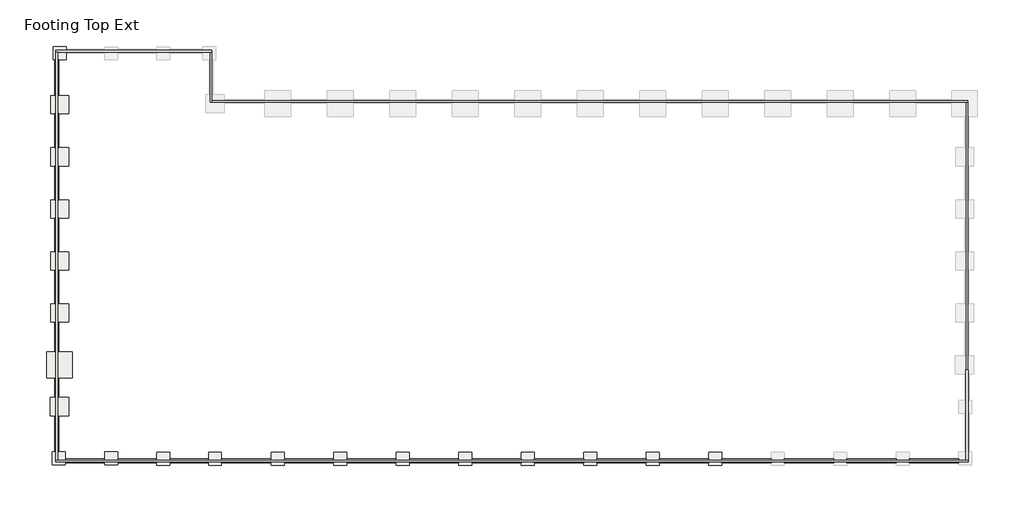
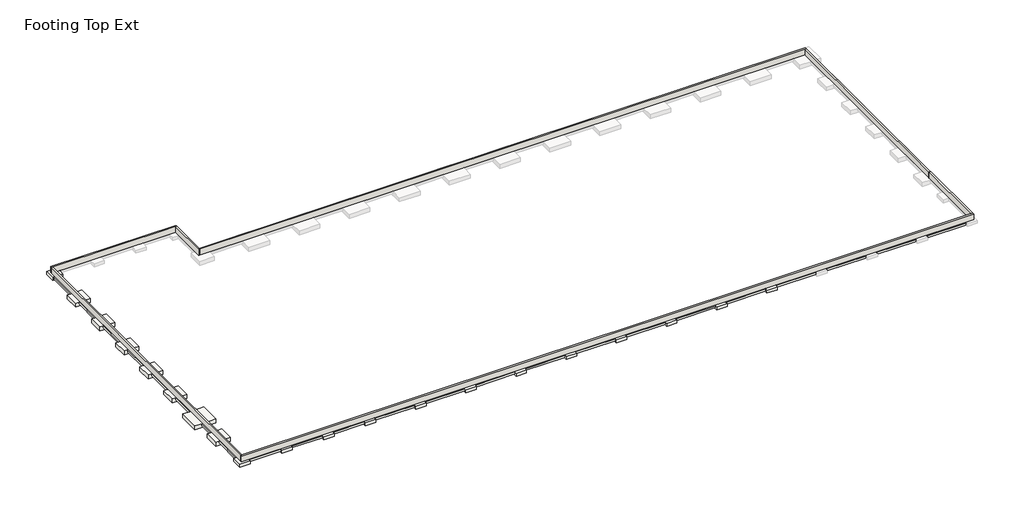
# One storey, part 1 of 2: 20 slabs, 7 walls, 2 footings.
"""IFC4 building model written with IfcOpenShell, lengths in millimetres."""

from ifc_helpers import new_model, si_unit, frame, origin, place, context, project, spatial, polyline, outline, extrude, faceted_brep, element, save

model = new_model("IFC4")

# Units and contexts
model_context = context("Model", 3, world=origin())
ifc_project = project(units=[si_unit("LENGTHUNIT", "METRE", prefix="MILLI")], contexts=[model_context])

# Site, building, storey
site = spatial("IfcSite", under=ifc_project)
building = spatial("IfcBuilding", under=site)
storey = spatial("IfcBuildingStorey", under=building, Name="Footing Top Ext", Elevation=-914.4)

# Footings
placement = place(None, origin())
element("IfcFooting", 1, ObjectType="Bearing Footing - 18\" x 12\"", at=placement, inside=storey, context=model_context, shape_type="SweptSolid", body=[
    extrude(outline(polyline([(305608.1398264, -579216.5913841), (305608.1398264, -578759.3913841), (310230.9398264, -578759.3913841), (310230.9398264, -579216.5913841), (305608.1398264, -579216.5913841)])), frame((0.0, 0.0, -1219.2), z_axis=(0.0, 0.0, 1.0), x_axis=(1.0, 0.0, 0.0)), (0.0, 0.0, 1.0), 304.8),
    extrude(outline(polyline([(311754.9398264, -579216.5913841), (311754.9398264, -578759.3913841), (316361.8648264, -578759.3913841), (316361.8648264, -579216.5913841), (311754.9398264, -579216.5913841)])), frame((0.0, 0.0, -1219.2), z_axis=(0.0, 0.0, 1.0), x_axis=(1.0, 0.0, 0.0)), (0.0, 0.0, 1.0), 304.8),
    extrude(outline(polyline([(317885.8648264, -579216.5913841), (317885.8648264, -578759.3913841), (322457.8648264, -578759.3913841), (322457.8648264, -579216.5913841), (317885.8648264, -579216.5913841)])), frame((0.0, 0.0, -1219.2), z_axis=(0.0, 0.0, 1.0), x_axis=(1.0, 0.0, 0.0)), (0.0, 0.0, 1.0), 304.8),
    extrude(outline(polyline([(323981.8648264, -579216.5913841), (323981.8648264, -578759.3913841), (329839.7398264, -578759.3913841), (329839.7398264, -579216.5913841), (323981.8648264, -579216.5913841)])), frame((0.0, 0.0, -1219.2), z_axis=(0.0, 0.0, 1.0), x_axis=(1.0, 0.0, 0.0)), (0.0, 0.0, 1.0), 304.8),
    extrude(outline(polyline([(331363.7398264, -579216.5913841), (331363.7398264, -578759.3913841), (337193.0398264, -578759.3913841), (337193.0398264, -579216.5913841), (331363.7398264, -579216.5913841)])), frame((0.0, 0.0, -1219.2), z_axis=(0.0, 0.0, 1.0), x_axis=(1.0, 0.0, 0.0)), (0.0, 0.0, 1.0), 304.8),
    extrude(outline(polyline([(338717.0398264, -579216.5913841), (338717.0398264, -578759.3913841), (344546.3398264, -578759.3913841), (344546.3398264, -579216.5913841), (338717.0398264, -579216.5913841)])), frame((0.0, 0.0, -1219.2), z_axis=(0.0, 0.0, 1.0), x_axis=(1.0, 0.0, 0.0)), (0.0, 0.0, 1.0), 304.8),
    extrude(outline(polyline([(346070.3398264, -579216.5913841), (346070.3398264, -578759.3913841), (351899.6398264, -578759.3913841), (351899.6398264, -579216.5913841), (346070.3398264, -579216.5913841)])), frame((0.0, 0.0, -1219.2), z_axis=(0.0, 0.0, 1.0), x_axis=(1.0, 0.0, 0.0)), (0.0, 0.0, 1.0), 304.8),
    extrude(outline(polyline([(353423.6398264, -579216.5913841), (353423.6398264, -578759.3913841), (359252.9398264, -578759.3913841), (359252.9398264, -579216.5913841), (353423.6398264, -579216.5913841)])), frame((0.0, 0.0, -1219.2), z_axis=(0.0, 0.0, 1.0), x_axis=(1.0, 0.0, 0.0)), (0.0, 0.0, 1.0), 304.8),
    extrude(outline(polyline([(360776.9398264, -579216.5913841), (360776.9398264, -578759.3913841), (366606.2398264, -578759.3913841), (366606.2398264, -579216.5913841), (360776.9398264, -579216.5913841)])), frame((0.0, 0.0, -1219.2), z_axis=(0.0, 0.0, 1.0), x_axis=(1.0, 0.0, 0.0)), (0.0, 0.0, 1.0), 304.8),
    extrude(outline(polyline([(368130.2398264, -579216.5913841), (368130.2398264, -578759.3913841), (373959.5398264, -578759.3913841), (373959.5398264, -579216.5913841), (368130.2398264, -579216.5913841)])), frame((0.0, 0.0, -1219.2), z_axis=(0.0, 0.0, 1.0), x_axis=(1.0, 0.0, 0.0)), (0.0, 0.0, 1.0), 304.8),
    extrude(outline(polyline([(375483.5398264, -579216.5913841), (375483.5398264, -578759.3913841), (381312.8398264, -578759.3913841), (381312.8398264, -579216.5913841), (375483.5398264, -579216.5913841)])), frame((0.0, 0.0, -1219.2), z_axis=(0.0, 0.0, 1.0), x_axis=(1.0, 0.0, 0.0)), (0.0, 0.0, 1.0), 304.8),
    extrude(outline(polyline([(382836.8398264, -579216.5913841), (382836.8398264, -578759.3913841), (388666.1398264, -578759.3913841), (388666.1398264, -579216.5913841), (382836.8398264, -579216.5913841)])), frame((0.0, 0.0, -1219.2), z_axis=(0.0, 0.0, 1.0), x_axis=(1.0, 0.0, 0.0)), (0.0, 0.0, 1.0), 304.8),
    extrude(outline(polyline([(390190.1398264, -579216.5913841), (390190.1398264, -578759.3913841), (396019.4398264, -578759.3913841), (396019.4398264, -579216.5913841), (390190.1398264, -579216.5913841)])), frame((0.0, 0.0, -1219.2), z_axis=(0.0, 0.0, 1.0), x_axis=(1.0, 0.0, 0.0)), (0.0, 0.0, 1.0), 304.8),
    extrude(outline(polyline([(397543.4398264, -579216.5913841), (397543.4398264, -578759.3913841), (403372.7398264, -578759.3913841), (403372.7398264, -579216.5913841), (397543.4398264, -579216.5913841)])), frame((0.0, 0.0, -1219.2), z_axis=(0.0, 0.0, 1.0), x_axis=(1.0, 0.0, 0.0)), (0.0, 0.0, 1.0), 304.8),
    extrude(outline(polyline([(404896.7398264, -579216.5913841), (404896.7398264, -578759.3913841), (410700.6398264, -578759.3913841), (410700.6398264, -579216.5913841), (404896.7398264, -579216.5913841)])), frame((0.0, 0.0, -1219.2), z_axis=(0.0, 0.0, 1.0), x_axis=(1.0, 0.0, 0.0)), (0.0, 0.0, 1.0), 304.8),
])
element("IfcFooting", 2, ObjectType="Bearing Footing - 18\" x 12\"", at=placement, inside=storey, context=model_context, shape_type="SweptSolid", body=[
    extrude(outline(polyline([(304369.8898264, -531712.2413841), (304827.0898264, -531712.2413841), (304827.0898264, -535985.7913841), (304369.8898264, -535985.7913841), (304369.8898264, -531712.2413841)])), frame((0.0, 0.0, -1219.2), z_axis=(0.0, 0.0, 1.0), x_axis=(1.0, 0.0, 0.0)), (0.0, 0.0, 1.0), 304.8),
    extrude(outline(polyline([(304369.8898264, -538119.3913841), (304827.0898264, -538119.3913841), (304827.0898264, -542113.5413841), (304369.8898264, -542113.5413841), (304369.8898264, -538119.3913841)])), frame((0.0, 0.0, -1219.2), z_axis=(0.0, 0.0, 1.0), x_axis=(1.0, 0.0, 0.0)), (0.0, 0.0, 1.0), 304.8),
    extrude(outline(polyline([(304369.8898264, -544247.1413841), (304827.0898264, -544247.1413841), (304827.0898264, -548241.2913841), (304369.8898264, -548241.2913841), (304369.8898264, -544247.1413841)])), frame((0.0, 0.0, -1219.2), z_axis=(0.0, 0.0, 1.0), x_axis=(1.0, 0.0, 0.0)), (0.0, 0.0, 1.0), 304.8),
    extrude(outline(polyline([(304369.8898264, -550374.8913841), (304827.0898264, -550374.8913841), (304827.0898264, -554369.0413841), (304369.8898264, -554369.0413841), (304369.8898264, -550374.8913841)])), frame((0.0, 0.0, -1219.2), z_axis=(0.0, 0.0, 1.0), x_axis=(1.0, 0.0, 0.0)), (0.0, 0.0, 1.0), 304.8),
    extrude(outline(polyline([(304369.8898264, -556502.6413841), (304827.0898264, -556502.6413841), (304827.0898264, -560496.7913841), (304369.8898264, -560496.7913841), (304369.8898264, -556502.6413841)])), frame((0.0, 0.0, -1219.2), z_axis=(0.0, 0.0, 1.0), x_axis=(1.0, 0.0, 0.0)), (0.0, 0.0, 1.0), 304.8),
    extrude(outline(polyline([(304369.8898264, -562630.3913841), (304827.0898264, -562630.3913841), (304827.0898264, -566167.3413841), (304369.8898264, -566167.3413841), (304369.8898264, -562630.3913841)])), frame((0.0, 0.0, -1219.2), z_axis=(0.0, 0.0, 1.0), x_axis=(1.0, 0.0, 0.0)), (0.0, 0.0, 1.0), 304.8),
    extrude(outline(polyline([(304369.8898264, -569215.3413841), (304827.0898264, -569215.3413841), (304827.0898264, -571526.7413841), (304369.8898264, -571526.7413841), (304369.8898264, -569215.3413841)])), frame((0.0, 0.0, -1219.2), z_axis=(0.0, 0.0, 1.0), x_axis=(1.0, 0.0, 0.0)), (0.0, 0.0, 1.0), 304.8),
    extrude(outline(polyline([(304369.8898264, -573660.3413841), (304827.0898264, -573660.3413841), (304827.0898264, -577933.8913841), (304369.8898264, -577933.8913841), (304369.8898264, -573660.3413841)])), frame((0.0, 0.0, -1219.2), z_axis=(0.0, 0.0, 1.0), x_axis=(1.0, 0.0, 0.0)), (0.0, 0.0, 1.0), 304.8),
])

# Slabs
element("IfcSlab", 3, ObjectType="Footing-Rectangular : F10", at=placement, inside=storey, context=model_context, shape_type="Brep", body=[
    faceted_brep([(306452.6898264, -566167.3413841, -914.4), (304827.0898264, -566167.3413841, -914.4), (304369.8898264, -566167.3413841, -914.4), (303404.6898264, -566167.3413841, -914.4), (303404.6898264, -569215.3413841, -914.4), (304369.8898264, -569215.3413841, -914.4), (304827.0898264, -569215.3413841, -914.4), (306452.6898264, -569215.3413841, -914.4), (306452.6898264, -566167.3413841, -1524.0), (306452.6898264, -569215.3413841, -1524.0), (303404.6898264, -569215.3413841, -1524.0), (303404.6898264, -566167.3413841, -1524.0)], [[[0, 1, 2, 3, 4, 5, 6, 7]], [[8, 9, 10, 11]], [[3, 2, 1, 0, 8, 11]], [[4, 3, 11, 10]], [[7, 6, 5, 4, 10, 9]], [[0, 7, 9, 8]]]),
])
element("IfcSlab", 4, ObjectType="Footing-Rectangular : F5", at=placement, inside=storey, context=model_context, shape_type="Brep", body=[
    faceted_brep([(305697.0398264, -530188.2413841, -914.4), (304173.0398264, -530188.2413841, -914.4), (304173.0398264, -531712.2413841, -914.4), (304369.8898264, -531712.2413841, -914.4), (304827.0898264, -531712.2413841, -914.4), (305697.0398264, -531712.2413841, -914.4), (305697.0398264, -530975.6413841, -914.4), (305697.0398264, -530518.4413841, -914.4), (305697.0398264, -530188.2413841, -1371.6), (305697.0398264, -531712.2413841, -1371.6), (304173.0398264, -531712.2413841, -1371.6), (304173.0398264, -530188.2413841, -1371.6)], [[[0, 1, 2, 3, 4, 5, 6, 7]], [[8, 9, 10, 11]], [[1, 0, 8, 11]], [[2, 1, 11, 10]], [[5, 4, 3, 2, 10, 9]], [[0, 7, 6, 5, 9, 8]]]),
])
element("IfcSlab", 5, ObjectType="Footing-Rectangular : F5", at=placement, inside=storey, context=model_context, shape_type="Brep", body=[
    faceted_brep([(305608.1398264, -577933.8913841, -914.4), (304827.0898264, -577933.8913841, -914.4), (304369.8898264, -577933.8913841, -914.4), (304084.1398264, -577933.8913841, -914.4), (304084.1398264, -579457.8913841, -914.4), (305608.1398264, -579457.8913841, -914.4), (305608.1398264, -579216.5913841, -914.4), (305608.1398264, -578759.3913841, -914.4), (305608.1398264, -577933.8913841, -1371.6), (305608.1398264, -579457.8913841, -1371.6), (304084.1398264, -579457.8913841, -1371.6), (304084.1398264, -577933.8913841, -1371.6)], [[[0, 1, 2, 3, 4, 5, 6, 7]], [[8, 9, 10, 11]], [[3, 2, 1, 0, 8, 11]], [[4, 3, 11, 10]], [[5, 4, 10, 9]], [[0, 7, 6, 5, 9, 8]]]),
])
element("IfcSlab", 6, ObjectType="Footing-Rectangular : F5", at=placement, inside=storey, context=model_context, shape_type="Brep", body=[
    faceted_brep([(311754.9398264, -577927.5413841, -914.4), (310230.9398264, -577927.5413841, -914.4), (310230.9398264, -578759.3913841, -914.4), (310230.9398264, -579216.5913841, -914.4), (310230.9398264, -579451.5413841, -914.4), (311754.9398264, -579451.5413841, -914.4), (311754.9398264, -579216.5913841, -914.4), (311754.9398264, -578759.3913841, -914.4), (311754.9398264, -577927.5413841, -1371.6), (311754.9398264, -579451.5413841, -1371.6), (310230.9398264, -579451.5413841, -1371.6), (310230.9398264, -577927.5413841, -1371.6)], [[[0, 1, 2, 3, 4, 5, 6, 7]], [[8, 9, 10, 11]], [[1, 0, 8, 11]], [[4, 3, 2, 1, 11, 10]], [[5, 4, 10, 9]], [[0, 7, 6, 5, 9, 8]]]),
])
element("IfcSlab", 7, ObjectType="Footing-Rectangular : F5", at=placement, inside=storey, context=model_context, shape_type="Brep", body=[
    faceted_brep([(317885.8648264, -577971.9913841, -914.4), (316361.8648264, -577971.9913841, -914.4), (316361.8648264, -578759.3913841, -914.4), (316361.8648264, -579216.5913841, -914.4), (316361.8648264, -579495.9913841, -914.4), (317885.8648264, -579495.9913841, -914.4), (317885.8648264, -579216.5913841, -914.4), (317885.8648264, -578759.3913841, -914.4), (317885.8648264, -577971.9913841, -1371.6), (317885.8648264, -579495.9913841, -1371.6), (316361.8648264, -579495.9913841, -1371.6), (316361.8648264, -577971.9913841, -1371.6)], [[[0, 1, 2, 3, 4, 5, 6, 7]], [[8, 9, 10, 11]], [[1, 0, 8, 11]], [[4, 3, 2, 1, 11, 10]], [[5, 4, 10, 9]], [[0, 7, 6, 5, 9, 8]]]),
])
element("IfcSlab", 8, ObjectType="Footing-Rectangular : F5", at=placement, inside=storey, context=model_context, shape_type="Brep", body=[
    faceted_brep([(323981.8648264, -577971.9913841, -914.4), (322457.8648264, -577971.9913841, -914.4), (322457.8648264, -578759.3913841, -914.4), (322457.8648264, -579216.5913841, -914.4), (322457.8648264, -579495.9913841, -914.4), (323981.8648264, -579495.9913841, -914.4), (323981.8648264, -579216.5913841, -914.4), (323981.8648264, -578759.3913841, -914.4), (323981.8648264, -577971.9913841, -1371.6), (323981.8648264, -579495.9913841, -1371.6), (322457.8648264, -579495.9913841, -1371.6), (322457.8648264, -577971.9913841, -1371.6)], [[[0, 1, 2, 3, 4, 5, 6, 7]], [[8, 9, 10, 11]], [[1, 0, 8, 11]], [[4, 3, 2, 1, 11, 10]], [[5, 4, 10, 9]], [[0, 7, 6, 5, 9, 8]]]),
])
element("IfcSlab", 9, ObjectType="Footing-Rectangular : F5", at=placement, inside=storey, context=model_context, shape_type="Brep", body=[
    faceted_brep([(331363.7398264, -577978.3413841, -914.4), (329839.7398264, -577978.3413841, -914.4), (329839.7398264, -578759.3913841, -914.4), (329839.7398264, -579216.5913841, -914.4), (329839.7398264, -579502.3413841, -914.4), (331363.7398264, -579502.3413841, -914.4), (331363.7398264, -579216.5913841, -914.4), (331363.7398264, -578759.3913841, -914.4), (331363.7398264, -577978.3413841, -1371.6), (331363.7398264, -579502.3413841, -1371.6), (329839.7398264, -579502.3413841, -1371.6), (329839.7398264, -577978.3413841, -1371.6)], [[[0, 1, 2, 3, 4, 5, 6, 7]], [[8, 9, 10, 11]], [[1, 0, 8, 11]], [[4, 3, 2, 1, 11, 10]], [[5, 4, 10, 9]], [[0, 7, 6, 5, 9, 8]]]),
])
element("IfcSlab", 10, ObjectType="Footing-Rectangular : F5", at=placement, inside=storey, context=model_context, shape_type="Brep", body=[
    faceted_brep([(338717.0398264, -577978.3413841, -914.4), (337193.0398264, -577978.3413841, -914.4), (337193.0398264, -578759.3913841, -914.4), (337193.0398264, -579216.5913841, -914.4), (337193.0398264, -579502.3413841, -914.4), (338717.0398264, -579502.3413841, -914.4), (338717.0398264, -579216.5913841, -914.4), (338717.0398264, -578759.3913841, -914.4), (338717.0398264, -577978.3413841, -1371.6), (338717.0398264, -579502.3413841, -1371.6), (337193.0398264, -579502.3413841, -1371.6), (337193.0398264, -577978.3413841, -1371.6)], [[[0, 1, 2, 3, 4, 5, 6, 7]], [[8, 9, 10, 11]], [[1, 0, 8, 11]], [[4, 3, 2, 1, 11, 10]], [[5, 4, 10, 9]], [[0, 7, 6, 5, 9, 8]]]),
])
element("IfcSlab", 11, ObjectType="Footing-Rectangular : F5", at=placement, inside=storey, context=model_context, shape_type="Brep", body=[
    faceted_brep([(346070.3398264, -577978.3413841, -914.4), (344546.3398264, -577978.3413841, -914.4), (344546.3398264, -578759.3913841, -914.4), (344546.3398264, -579216.5913841, -914.4), (344546.3398264, -579502.3413841, -914.4), (346070.3398264, -579502.3413841, -914.4), (346070.3398264, -579216.5913841, -914.4), (346070.3398264, -578759.3913841, -914.4), (346070.3398264, -577978.3413841, -1371.6), (346070.3398264, -579502.3413841, -1371.6), (344546.3398264, -579502.3413841, -1371.6), (344546.3398264, -577978.3413841, -1371.6)], [[[0, 1, 2, 3, 4, 5, 6, 7]], [[8, 9, 10, 11]], [[1, 0, 8, 11]], [[4, 3, 2, 1, 11, 10]], [[5, 4, 10, 9]], [[0, 7, 6, 5, 9, 8]]]),
])
element("IfcSlab", 12, ObjectType="Footing-Rectangular : F5", at=placement, inside=storey, context=model_context, shape_type="Brep", body=[
    faceted_brep([(353423.6398264, -577978.3413841, -914.4), (351899.6398264, -577978.3413841, -914.4), (351899.6398264, -578759.3913841, -914.4), (351899.6398264, -579216.5913841, -914.4), (351899.6398264, -579502.3413841, -914.4), (353423.6398264, -579502.3413841, -914.4), (353423.6398264, -579216.5913841, -914.4), (353423.6398264, -578759.3913841, -914.4), (353423.6398264, -577978.3413841, -1371.6), (353423.6398264, -579502.3413841, -1371.6), (351899.6398264, -579502.3413841, -1371.6), (351899.6398264, -577978.3413841, -1371.6)], [[[0, 1, 2, 3, 4, 5, 6, 7]], [[8, 9, 10, 11]], [[1, 0, 8, 11]], [[4, 3, 2, 1, 11, 10]], [[5, 4, 10, 9]], [[0, 7, 6, 5, 9, 8]]]),
])
element("IfcSlab", 13, ObjectType="Footing-Rectangular : F5", at=placement, inside=storey, context=model_context, shape_type="Brep", body=[
    faceted_brep([(360776.9398264, -577978.3413841, -914.4), (359252.9398264, -577978.3413841, -914.4), (359252.9398264, -578759.3913841, -914.4), (359252.9398264, -579216.5913841, -914.4), (359252.9398264, -579502.3413841, -914.4), (360776.9398264, -579502.3413841, -914.4), (360776.9398264, -579216.5913841, -914.4), (360776.9398264, -578759.3913841, -914.4), (360776.9398264, -577978.3413841, -1371.6), (360776.9398264, -579502.3413841, -1371.6), (359252.9398264, -579502.3413841, -1371.6), (359252.9398264, -577978.3413841, -1371.6)], [[[0, 1, 2, 3, 4, 5, 6, 7]], [[8, 9, 10, 11]], [[1, 0, 8, 11]], [[4, 3, 2, 1, 11, 10]], [[5, 4, 10, 9]], [[0, 7, 6, 5, 9, 8]]]),
])
element("IfcSlab", 14, ObjectType="Footing-Rectangular : F5", at=placement, inside=storey, context=model_context, shape_type="Brep", body=[
    faceted_brep([(368130.2398264, -577978.3413841, -914.4), (366606.2398264, -577978.3413841, -914.4), (366606.2398264, -578759.3913841, -914.4), (366606.2398264, -579216.5913841, -914.4), (366606.2398264, -579502.3413841, -914.4), (368130.2398264, -579502.3413841, -914.4), (368130.2398264, -579216.5913841, -914.4), (368130.2398264, -578759.3913841, -914.4), (368130.2398264, -577978.3413841, -1371.6), (368130.2398264, -579502.3413841, -1371.6), (366606.2398264, -579502.3413841, -1371.6), (366606.2398264, -577978.3413841, -1371.6)], [[[0, 1, 2, 3, 4, 5, 6, 7]], [[8, 9, 10, 11]], [[1, 0, 8, 11]], [[4, 3, 2, 1, 11, 10]], [[5, 4, 10, 9]], [[0, 7, 6, 5, 9, 8]]]),
])
element("IfcSlab", 15, ObjectType="Footing-Rectangular : F5", at=placement, inside=storey, context=model_context, shape_type="Brep", body=[
    faceted_brep([(375483.5398264, -577978.3413841, -914.4), (373959.5398264, -577978.3413841, -914.4), (373959.5398264, -578759.3913841, -914.4), (373959.5398264, -579216.5913841, -914.4), (373959.5398264, -579502.3413841, -914.4), (375483.5398264, -579502.3413841, -914.4), (375483.5398264, -579216.5913841, -914.4), (375483.5398264, -578759.3913841, -914.4), (375483.5398264, -577978.3413841, -1371.6), (375483.5398264, -579502.3413841, -1371.6), (373959.5398264, -579502.3413841, -1371.6), (373959.5398264, -577978.3413841, -1371.6)], [[[0, 1, 2, 3, 4, 5, 6, 7]], [[8, 9, 10, 11]], [[1, 0, 8, 11]], [[4, 3, 2, 1, 11, 10]], [[5, 4, 10, 9]], [[0, 7, 6, 5, 9, 8]]]),
])
element("IfcSlab", 16, ObjectType="Footing-Rectangular : F5", at=placement, inside=storey, context=model_context, shape_type="Brep", body=[
    faceted_brep([(382836.8398264, -577978.3413841, -914.4), (381312.8398264, -577978.3413841, -914.4), (381312.8398264, -578759.3913841, -914.4), (381312.8398264, -579216.5913841, -914.4), (381312.8398264, -579502.3413841, -914.4), (382836.8398264, -579502.3413841, -914.4), (382836.8398264, -579216.5913841, -914.4), (382836.8398264, -578759.3913841, -914.4), (382836.8398264, -577978.3413841, -1371.6), (382836.8398264, -579502.3413841, -1371.6), (381312.8398264, -579502.3413841, -1371.6), (381312.8398264, -577978.3413841, -1371.6)], [[[0, 1, 2, 3, 4, 5, 6, 7]], [[8, 9, 10, 11]], [[1, 0, 8, 11]], [[4, 3, 2, 1, 11, 10]], [[5, 4, 10, 9]], [[0, 7, 6, 5, 9, 8]]]),
])
element("IfcSlab", 17, ObjectType="Footing-Rectangular : F7", at=placement, inside=storey, context=model_context, shape_type="Brep", body=[
    faceted_brep([(306020.8898264, -535985.7913841, -914.4), (304827.0898264, -535985.7913841, -914.4), (304369.8898264, -535985.7913841, -914.4), (303887.2898264, -535985.7913841, -914.4), (303887.2898264, -538119.3913841, -914.4), (304369.8898264, -538119.3913841, -914.4), (304827.0898264, -538119.3913841, -914.4), (306020.8898264, -538119.3913841, -914.4), (306020.8898264, -535985.7913841, -1524.0), (306020.8898264, -538119.3913841, -1524.0), (303887.2898264, -538119.3913841, -1524.0), (303887.2898264, -535985.7913841, -1524.0)], [[[0, 1, 2, 3, 4, 5, 6, 7]], [[8, 9, 10, 11]], [[3, 2, 1, 0, 8, 11]], [[4, 3, 11, 10]], [[7, 6, 5, 4, 10, 9]], [[0, 7, 9, 8]]]),
])
element("IfcSlab", 18, ObjectType="Footing-Rectangular : F7", at=placement, inside=storey, context=model_context, shape_type="Brep", body=[
    faceted_brep([(306020.8898264, -542113.5413841, -914.4), (304827.0898264, -542113.5413841, -914.4), (304369.8898264, -542113.5413841, -914.4), (303887.2898264, -542113.5413841, -914.4), (303887.2898264, -544247.1413841, -914.4), (304369.8898264, -544247.1413841, -914.4), (304827.0898264, -544247.1413841, -914.4), (306020.8898264, -544247.1413841, -914.4), (306020.8898264, -542113.5413841, -1524.0), (306020.8898264, -544247.1413841, -1524.0), (303887.2898264, -544247.1413841, -1524.0), (303887.2898264, -542113.5413841, -1524.0)], [[[0, 1, 2, 3, 4, 5, 6, 7]], [[8, 9, 10, 11]], [[3, 2, 1, 0, 8, 11]], [[4, 3, 11, 10]], [[7, 6, 5, 4, 10, 9]], [[0, 7, 9, 8]]]),
])
element("IfcSlab", 19, ObjectType="Footing-Rectangular : F7", at=placement, inside=storey, context=model_context, shape_type="Brep", body=[
    faceted_brep([(306020.8898264, -548241.2913841, -914.4), (304827.0898264, -548241.2913841, -914.4), (304369.8898264, -548241.2913841, -914.4), (303887.2898264, -548241.2913841, -914.4), (303887.2898264, -550374.8913841, -914.4), (304369.8898264, -550374.8913841, -914.4), (304827.0898264, -550374.8913841, -914.4), (306020.8898264, -550374.8913841, -914.4), (306020.8898264, -548241.2913841, -1524.0), (306020.8898264, -550374.8913841, -1524.0), (303887.2898264, -550374.8913841, -1524.0), (303887.2898264, -548241.2913841, -1524.0)], [[[0, 1, 2, 3, 4, 5, 6, 7]], [[8, 9, 10, 11]], [[3, 2, 1, 0, 8, 11]], [[4, 3, 11, 10]], [[7, 6, 5, 4, 10, 9]], [[0, 7, 9, 8]]]),
])
element("IfcSlab", 20, ObjectType="Footing-Rectangular : F7", at=placement, inside=storey, context=model_context, shape_type="Brep", body=[
    faceted_brep([(306020.8898264, -554369.0413841, -914.4), (304827.0898264, -554369.0413841, -914.4), (304369.8898264, -554369.0413841, -914.4), (303887.2898264, -554369.0413841, -914.4), (303887.2898264, -556502.6413841, -914.4), (304369.8898264, -556502.6413841, -914.4), (304827.0898264, -556502.6413841, -914.4), (306020.8898264, -556502.6413841, -914.4), (306020.8898264, -554369.0413841, -1524.0), (306020.8898264, -556502.6413841, -1524.0), (303887.2898264, -556502.6413841, -1524.0), (303887.2898264, -554369.0413841, -1524.0)], [[[0, 1, 2, 3, 4, 5, 6, 7]], [[8, 9, 10, 11]], [[3, 2, 1, 0, 8, 11]], [[4, 3, 11, 10]], [[7, 6, 5, 4, 10, 9]], [[0, 7, 9, 8]]]),
])
element("IfcSlab", 21, ObjectType="Footing-Rectangular : F7", at=placement, inside=storey, context=model_context, shape_type="Brep", body=[
    faceted_brep([(306020.8898264, -560496.7913841, -914.4), (304827.0898264, -560496.7913841, -914.4), (304369.8898264, -560496.7913841, -914.4), (303887.2898264, -560496.7913841, -914.4), (303887.2898264, -562630.3913841, -914.4), (304369.8898264, -562630.3913841, -914.4), (304827.0898264, -562630.3913841, -914.4), (306020.8898264, -562630.3913841, -914.4), (306020.8898264, -560496.7913841, -1524.0), (306020.8898264, -562630.3913841, -1524.0), (303887.2898264, -562630.3913841, -1524.0), (303887.2898264, -560496.7913841, -1524.0)], [[[0, 1, 2, 3, 4, 5, 6, 7]], [[8, 9, 10, 11]], [[3, 2, 1, 0, 8, 11]], [[4, 3, 11, 10]], [[7, 6, 5, 4, 10, 9]], [[0, 7, 9, 8]]]),
])
element("IfcSlab", 22, ObjectType="Footing-Rectangular : F7", at=placement, inside=storey, context=model_context, shape_type="Brep", body=[
    faceted_brep([(305995.4898264, -571526.7413841, -914.4), (304827.0898264, -571526.7413841, -914.4), (304369.8898264, -571526.7413841, -914.4), (303861.8898264, -571526.7413841, -914.4), (303861.8898264, -573660.3413841, -914.4), (304369.8898264, -573660.3413841, -914.4), (304827.0898264, -573660.3413841, -914.4), (305995.4898264, -573660.3413841, -914.4), (305995.4898264, -571526.7413841, -1524.0), (305995.4898264, -573660.3413841, -1524.0), (303861.8898264, -573660.3413841, -1524.0), (303861.8898264, -571526.7413841, -1524.0)], [[[0, 1, 2, 3, 4, 5, 6, 7]], [[8, 9, 10, 11]], [[3, 2, 1, 0, 8, 11]], [[4, 3, 11, 10]], [[7, 6, 5, 4, 10, 9]], [[0, 7, 9, 8]]]),
])

# Walls
element("IfcWall", 23, ObjectType="Frost Wall - 12\" Concrete", at=placement, inside=storey, context=model_context, shape_type="SweptSolid", body=[
    extrude(outline(polyline([(411551.5398264, -578886.3913841), (411551.5398264, -568288.2413841), (411856.3398264, -568288.2413841), (411856.3398264, -578886.3913841), (411551.5398264, -578886.3913841)])), frame((0.0, 0.0, -914.4), z_axis=(0.0, 0.0, 1.0), x_axis=(1.0, 0.0, 0.0)), (0.0, 0.0, 1.0), 914.4),
])
element("IfcWall", 24, ObjectType="Frost Wall - 8\" Concrete", at=placement, inside=storey, context=model_context, shape_type="Brep", body=[
    faceted_brep([(304496.8898264, -530848.6413841, -914.4), (304700.0898264, -530848.6413841, -914.4), (322664.2398264, -530848.6413841, -914.4), (322867.4398264, -530848.6413841, -914.4), (322867.4398264, -530848.6413841, 0.0), (322664.2398264, -530848.6413841, 0.0), (304700.0898264, -530848.6413841, 0.0), (304496.8898264, -530848.6413841, 0.0), (304496.8898264, -530645.4413841, -914.4), (304496.8898264, -530645.4413841, 0.0), (322867.4398264, -530645.4413841, 0.0), (322867.4398264, -530645.4413841, -914.4)], [[[0, 1, 2, 3, 4, 5, 6, 7]], [[8, 9, 10, 11]], [[3, 2, 1, 0, 8, 11]], [[7, 6, 5, 4, 10, 9]], [[4, 3, 11, 10]], [[0, 7, 9, 8]]]),
])
element("IfcWall", 25, ObjectType="Frost Wall - 8\" Concrete", at=placement, inside=storey, context=model_context, shape_type="Brep", body=[
    faceted_brep([(322664.2398264, -530848.6413841, -914.4), (322664.2398264, -536760.4913841, -914.4), (322664.2398264, -536760.4913841, -152.4), (322664.2398264, -536760.4913841, 0.0), (322664.2398264, -530848.6413841, 0.0), (322664.2398264, -530848.6413841, -152.4), (322867.4398264, -536760.4913841, -914.4), (322867.4398264, -536557.2913841, -914.4), (322867.4398264, -530848.6413841, -914.4), (322867.4398264, -530848.6413841, 0.0), (322867.4398264, -536557.2913841, 0.0), (322867.4398264, -536760.4913841, 0.0), (322867.4398264, -536760.4913841, -152.4)], [[[0, 1, 2, 3, 4, 5]], [[6, 7, 8, 9, 10, 11, 12]], [[1, 0, 8, 7, 6]], [[4, 3, 11, 10, 9]], [[4, 9, 8, 0, 5]], [[1, 6, 12, 11, 3, 2]]]),
])
element("IfcWall", 26, ObjectType="Frost Wall - 8\" Concrete", at=placement, inside=storey, context=model_context, shape_type="Brep", body=[
    faceted_brep([(322867.4398264, -536760.4913841, -914.4), (411564.2398264, -536760.4913841, -914.4), (411767.4398264, -536760.4913841, -914.4), (411767.4398264, -536760.4913841, 0.0), (411564.2398264, -536760.4913841, 0.0), (322867.4398264, -536760.4913841, 0.0), (322867.4398264, -536760.4913841, -152.4), (411767.4398264, -536557.2913841, -914.4), (322867.4398264, -536557.2913841, -914.4), (322867.4398264, -536557.2913841, 0.0), (411767.4398264, -536557.2913841, 0.0)], [[[0, 1, 2, 3, 4, 5, 6]], [[7, 8, 9, 10]], [[2, 1, 0, 8, 7]], [[10, 9, 5, 4, 3]], [[5, 9, 8, 0, 6]], [[3, 2, 7, 10]]]),
])
element("IfcWall", 27, ObjectType="Frost Wall - 8\" Concrete", at=placement, inside=storey, context=model_context, shape_type="SweptSolid", body=[
    extrude(outline(polyline([(411564.2398264, -568288.2413841), (411564.2398264, -536760.4913841), (411767.4398264, -536760.4913841), (411767.4398264, -568288.2413841), (411564.2398264, -568288.2413841)])), frame((0.0, 0.0, -914.4), z_axis=(0.0, 0.0, 1.0), x_axis=(1.0, 0.0, 0.0)), (0.0, 0.0, 1.0), 914.4),
])
element("IfcWall", 28, ObjectType="Frost Wall - 8\" Concrete", at=placement, inside=storey, context=model_context, shape_type="Brep", body=[
    faceted_brep([(411856.3398264, -578886.3913841, -914.4), (411551.5398264, -578886.3913841, -914.4), (304700.0898264, -578886.3913841, -914.4), (304496.8898264, -578886.3913841, -914.4), (304496.8898264, -578886.3913841, 0.0), (304700.0898264, -578886.3913841, 0.0), (357559.8710764, -578886.3913841, 0.0), (359693.4710764, -578886.3913841, 0.0), (387023.0773264, -578886.3913841, 0.0), (397962.5398264, -578886.3913841, 0.0), (404753.8648264, -578886.3913841, 0.0), (407192.2648264, -578886.3913841, 0.0), (411551.5398264, -578886.3913841, 0.0), (411856.3398264, -578886.3913841, 0.0), (411856.3398264, -579089.5913841, -914.4), (411856.3398264, -579089.5913841, 0.0), (304496.8898264, -579089.5913841, 0.0), (304496.8898264, -579089.5913841, -914.4)], [[[0, 1, 2, 3, 4, 5, 6, 7, 8, 9, 10, 11, 12, 13]], [[14, 15, 16, 17]], [[3, 2, 1, 0, 14, 17]], [[13, 12, 11, 10, 9, 8, 7, 6, 5, 4, 16, 15]], [[4, 3, 17, 16]], [[0, 13, 15, 14]]]),
])
element("IfcWall", 29, ObjectType="Frost Wall - 8\" Concrete", at=placement, inside=storey, context=model_context, shape_type="SweptSolid", body=[
    extrude(outline(polyline([(304700.0898264, -530848.6413841), (304700.0898264, -578886.3913841), (304496.8898264, -578886.3913841), (304496.8898264, -530848.6413841), (304700.0898264, -530848.6413841)])), frame((0.0, 0.0, -914.4), z_axis=(0.0, 0.0, 1.0), x_axis=(1.0, 0.0, 0.0)), (0.0, 0.0, 1.0), 914.4),
])

save(model, "model.ifc")

# Revit data of these elements
# Project information
#   Project Issue Date = "07/08/2015"
#   Project Status = "Project Status"
#   Client Name = "Xcel"
#   Project Address = "Enter address here"
#   Project Name = "Sports Complex"
#   Project Number = "Project Number"
# Grids (mm)
#   "2-A.G": line (303404.69, -579000.691) -> (412910.44, -579000.691)
#   "2-12": line (330601.74, -530188.241) -> (330601.74, -579502.341)
#   "2": line (330601.74, -462514.089) -> (330601.74, -614425.444)
#   "3": line (337955.04, -462514.089) -> (337955.04, -614425.444)
#   "4": line (310992.94, -462514.089) -> (310992.94, -614425.444)
#   "5": line (317120.69, -462514.089) -> (317120.69, -614425.444)
#   "6": line (304788.99, -466694.458) -> (304788.99, -614353.824)
#   "7": line (304585.79, -462514.089) -> (304585.79, -614425.444)
#   "8": line (323527.84, -456865.657) -> (323527.84, -614425.444)
#   "9": line (323324.64, -458611.498) -> (323324.64, -614425.444)
#   "10": line (323121.44, -459359.716) -> (323121.44, -614425.444)
#   "1-13.G ALT": line (322867.44, -459359.716) -> (322867.44, -614425.444)
#   "12": line (330601.74, -466694.458) -> (330601.74, -617473.444)
#   "13": line (337955.04, -466694.458) -> (337955.04, -617473.444)
#   "14": line (323324.64, -466694.458) -> (323324.64, -616559.044)
#   "3-D ALT": line (322664.24, -456865.657) -> (322664.24, -614425.444)
#   "3-D.G ALT": line (322867.44, -458611.498) -> (322867.44, -614425.444)
#   "1-12": line (330601.74, -530188.241) -> (330601.74, -579502.341)
#   "1-11": line (337955.04, -530188.241) -> (337955.04, -579502.341)
#   "1-10": line (345308.34, -530188.241) -> (345308.34, -579502.341)
#   "1-9": line (352661.64, -530188.241) -> (352661.64, -579502.341)
#   "1-8": line (360014.94, -530188.241) -> (360014.94, -579502.341)
#   "1-7": line (367368.24, -530188.241) -> (367368.24, -579502.341)
#   "3-7": line (303404.69, -543180.341) -> (412910.44, -543180.341)
#   "3-6": line (303404.69, -549308.091) -> (412910.44, -549308.091)
#   "1-6": line (374721.54, -530188.241) -> (374721.54, -579502.341)
#   "1-5": line (382074.84, -530188.241) -> (382074.84, -579502.341)
#   "1-4": line (389428.14, -530188.241) -> (389428.14, -579502.341)
#   "1-3": line (396781.44, -530188.241) -> (396781.44, -579502.341)
#   "1-2": line (404134.74, -530188.241) -> (404134.74, -579502.341)
#   "3-8": line (303404.69, -537052.591) -> (412910.44, -537052.591)
#   "3-3": line (303404.69, -567691.341) -> (412910.44, -567691.341)
#   "3-5": line (303404.69, -555435.841) -> (412910.44, -555435.841)
#   "3-4": line (303404.69, -561563.591) -> (412910.44, -561563.591)
#   "3-2": line (303404.69, -572593.541) -> (412910.44, -572593.541)
#   "3-B": line (310992.94, -530188.241) -> (310992.94, -579502.341)
#   "3-C": line (317120.69, -530188.241) -> (317120.69, -579502.341)
#   "3-1": line (303404.69, -578797.491) -> (412910.44, -578797.491)
#   "3-1.G": line (303404.69, -579000.691) -> (412910.44, -579000.691)
#   "3-A": line (304788.99, -530188.241) -> (304788.99, -579502.341)
#   "3-A.G": line (304585.79, -530188.241) -> (304585.79, -579502.341)
#   "3-9": line (303404.69, -530848.641) -> (412910.44, -530848.641)
#   "3-9.G": line (303404.69, -530645.441) -> (412910.44, -530645.441)
#   "3-E.G": line (323527.84, -530188.241) -> (323527.84, -579502.341)
#   "3-E": line (323324.64, -530188.241) -> (323324.64, -579502.341)
#   "3-3.G": line (303404.69, -567488.141) -> (412910.44, -567488.141)
#   "1-1G": line (411767.44, -530188.241) -> (411767.44, -579502.341)
#   "2-1": line (411513.44, -530188.241) -> (411513.44, -579502.341)
#   "1-1": line (411513.44, -530188.241) -> (411513.44, -579502.341)
#   "1-13": line (323121.44, -530188.241) -> (323121.44, -579502.341)
#   "1-A": line (303404.69, -567932.641) -> (412910.44, -567932.641)
#   "1-A.G": line (303404.69, -568186.641) -> (412910.44, -568186.641)
#   "1-13.G": line (322867.44, -530188.241) -> (322867.44, -579502.341)
#   "3-D": line (322664.24, -530188.241) -> (322664.24, -579502.341)
#   "1-F": line (303404.69, -536811.291) -> (412910.44, -536811.291)
#   "1-F.G": line (303404.69, -536557.291) -> (412910.44, -536557.291)
#   "3-D.G": line (322867.44, -530188.241) -> (322867.44, -579502.341)
#   "1-E": line (303404.69, -543180.341) -> (412910.44, -543180.341)
#   "1-D": line (303404.69, -549308.091) -> (412910.44, -549308.091)
#   "1-C": line (303404.69, -555435.841) -> (412910.44, -555435.841)
#   "1-B": line (303404.69, -561563.591) -> (412910.44, -561563.591)
#   "2-B": line (303404.69, -572593.541) -> (412910.44, -572593.541)
#   "2-A": line (303404.69, -578797.491) -> (412910.44, -578797.491)
#   "2-6": line (374721.54, -530188.241) -> (374721.54, -579502.341)
#   "2-5": line (382074.84, -530188.241) -> (382074.84, -579502.341)
#   "2-4": line (389428.14, -530188.241) -> (389428.14, -579502.341)
#   "2-3": line (396781.44, -530188.241) -> (396781.44, -579502.341)
#   "2-11": line (337955.04, -530188.241) -> (337955.04, -579502.341)
#   "2-10": line (345308.34, -530188.241) -> (345308.34, -579502.341)
#   "2-9": line (352661.64, -530188.241) -> (352661.64, -579502.341)
#   "2-8": line (360014.94, -530188.241) -> (360014.94, -579502.341)
#   "2-7": line (367368.24, -530188.241) -> (367368.24, -579502.341)
#   "2-2": line (404134.74, -530188.241) -> (404134.74, -579502.341)
#   "2-13": line (323324.64, -530188.241) -> (323324.64, -579502.341)
#   "2-1G": line (411767.44, -530188.241) -> (411767.44, -579502.341)
#   "2-C": line (303404.69, -567932.641) -> (412910.44, -567932.641)
#   "2-3.G": line (396578.24, -530188.241) -> (396578.24, -579502.341)
# Type "Bearing Footing - 18\" x 12\""
#   Assembly Code = "A1010110"
# Type "Footing-Rectangular : F10"
#   Assembly Code = "A1010100"
#   Width = 10' - 0"
#   Length = 10' - 0"
#   Thickness = 2' - 0"
#   Structural Material [instance default] = CONCRETE FOOTING - SEE STRUCT DWGS.
# Type "Footing-Rectangular : F5"
#   Assembly Code = "A1010100"
#   Width = 5' - 0"
#   Length = 5' - 0"
#   Thickness = 1' - 6"
#   Structural Material [instance default] = CONCRETE FOOTING - SEE STRUCT DWGS.
# Type "Footing-Rectangular : F7"
#   Assembly Code = "A1010100"
#   Width = 7' - 0"
#   Length = 7' - 0"
#   Thickness = 2' - 0"
#   Structural Material [instance default] = CONCRETE FOOTING - SEE STRUCT DWGS.
# Type "Frost Wall - 12\" Concrete"
#   Assembly Code = "B2010"
#   Layers, outside or top first: 1' - 0" "CONCRETE FROST WALL - SEE STRUCT DWGS." (function 1)
# Type "Frost Wall - 8\" Concrete"
#   Assembly Code = "B2010"
#   Layers, outside or top first: 0' - 8" "CONCRETE FROST WALL - SEE STRUCT DWGS." (function 1)
# Elements 1, 2 (IfcFooting, "Bearing Footing - 18\" x 12\"")
#   Phase Created = Existing
#   Materials on its faces: "CONCRETE FOOTING - SEE STRUCT DWGS."
# Element 3 (IfcSlab, "Footing-Rectangular : F10")
#   Comments = ""
#   Structural Material = CONCRETE FOOTING - SEE STRUCT DWGS.
#   Phase Created = Existing
#   Materials on its faces: "CONCRETE FOOTING - SEE STRUCT DWGS."
# Elements 4, 5, 6, 7, 8, 9, 10, 11, 12, 13, 14, 15, 16 (IfcSlab, "Footing-Rectangular : F5")
#   Comments = ""
#   Structural Material = CONCRETE FOOTING - SEE STRUCT DWGS.
#   Phase Created = Existing
#   Materials on its faces: "CONCRETE FOOTING - SEE STRUCT DWGS."
# Elements 17, 18, 19, 20, 21, 22 (IfcSlab, "Footing-Rectangular : F7")
#   Comments = ""
#   Structural Material = CONCRETE FOOTING - SEE STRUCT DWGS.
#   Phase Created = Existing
#   Materials on its faces: "CONCRETE FOOTING - SEE STRUCT DWGS."
# Element 23 (IfcWall, "Frost Wall - 12\" Concrete")
#   Comments = ""
#   Top Offset = 0' - 0"
#   Base Offset = 0' - 0"
#   wall height = 3' - 0"
#   Phase Created = Existing
#   Base Constraint = Footing Top Ext
#   Top Constraint = Level 1
#   Materials on its faces: "CONCRETE FROST WALL - SEE STRUCT DWGS."
# Elements 24, 25, 26, 27, 28, 29 (IfcWall, "Frost Wall - 8\" Concrete")
#   Comments = ""
#   Top Offset = 0' - 0"
#   Base Offset = 0' - 0"
#   wall height = 3' - 0"
#   Phase Created = Existing
#   Base Constraint = Footing Top Ext
#   Top Constraint = Level 1
#   Materials on its faces: "CONCRETE FROST WALL - SEE STRUCT DWGS."
# Materials
#   "CONCRETE FOOTING - SEE STRUCT DWGS.": class "Concrete", colour RGB 192 192 192, transparency 0, Description = "Cast-in-place concrete", Cost = 0
#   "CONCRETE FROST WALL - SEE STRUCT DWGS.": class "Concrete", colour RGB 192 192 192, transparency 0, Description = "Cast-in-place concrete", Cost = 0
